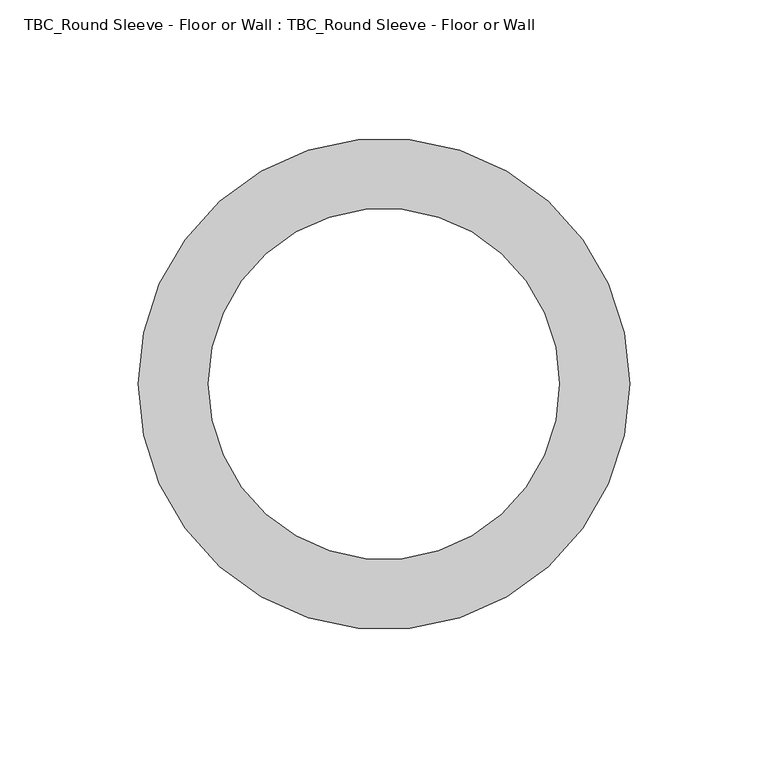
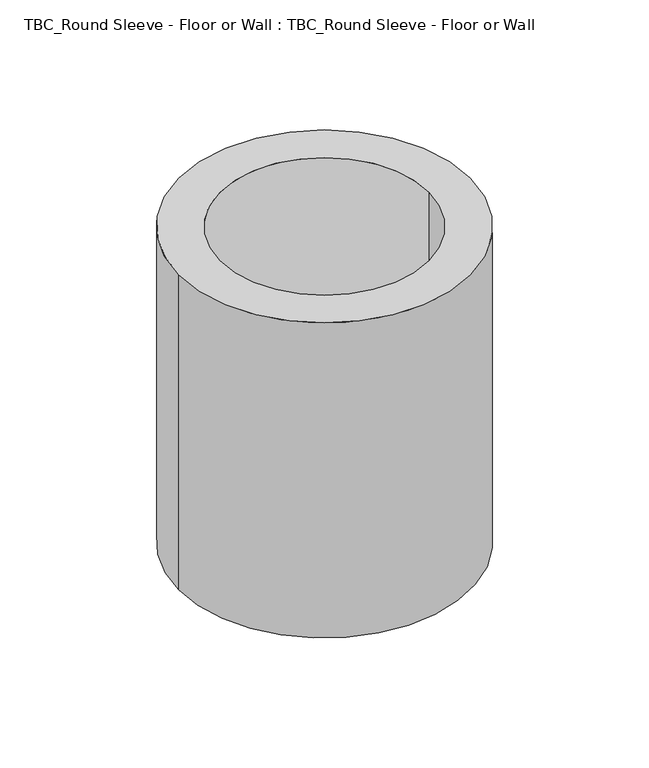
"""IFC4 building model written with IfcOpenShell, lengths in millimetres: proxy geometry, TBC_Round Sleeve - Floor or Wall : TBC_Round Sleeve - Floor or Wall."""

import ifcopenshell
import ifcopenshell.guid

model = None  # the IFC model being written
_history = None  # IfcOwnerHistory: only IFC2X3 demands one
_inside = {}  # id of a spatial element -> (the spatial element, [elements in it])
_under = {}  # id of a project, library or spatial element -> (it, [spatial elements below it])
_declared = {}  # id of a project -> (the project, [libraries it declares])
_typed = {}  # id of a type object -> (the type object, [elements of that type])
_made_of = {}  # id of a material, layer set ... -> (it, [elements and type objects made of it])


def new_model(schema):
    """Start an empty IFC model of exactly this schema.

    Asked for "IFC4X3", IfcOpenShell would pick the latest addendum, in which some entities
    have other attributes; the version numbers below select the first issue.
    IFC2X3 requires an IfcOwnerHistory on every rooted entity: one is made here for all.
    """
    global model, _history
    if schema == "IFC4X3":
        model = ifcopenshell.file(schema_version=(4, 3, 0, 0))
    else:
        model = ifcopenshell.file(schema=schema)
    _inside.clear()
    _under.clear()
    _declared.clear()
    _typed.clear()
    _made_of.clear()
    _history = None
    if model.schema == "IFC2X3":
        org = make("IfcOrganization", Name="unknown")
        user = make(
            "IfcPersonAndOrganization",
            ThePerson=make("IfcPerson", FamilyName="unknown"),
            TheOrganization=org,
        )
        app = make(
            "IfcApplication",
            ApplicationDeveloper=org,
            Version="unknown",
            ApplicationFullName="unknown",
            ApplicationIdentifier="unknown",
        )
        _history = make(
            "IfcOwnerHistory",
            OwningUser=user,
            OwningApplication=app,
            ChangeAction="ADDED",
            CreationDate=0,
        )
    return model


def make(cls, **values):
    """One entity of the class cls with the attributes given. An attribute that is None is left unset."""
    return model.create_entity(
        cls, **{name: value for name, value in values.items() if value is not None}
    )


def rooted(cls, **values):
    """An entity with a GlobalId (a new one), such as an element, a storey or a relation."""
    return make(cls, GlobalId=ifcopenshell.guid.new(), OwnerHistory=_history, **values)


def si_unit(unit_type, name, prefix=None):
    """IfcSIUnit, for example si_unit("LENGTHUNIT", "METRE", prefix="MILLI")."""
    return make("IfcSIUnit", UnitType=unit_type, Prefix=prefix, Name=name)


def assignment(units):
    """IfcUnitAssignment: the units of a project."""
    return None if units is None else make("IfcUnitAssignment", Units=units)


def point(xyz):
    """IfcCartesianPoint."""
    return None if xyz is None else make("IfcCartesianPoint", Coordinates=xyz)


def direction(xyz):
    """IfcDirection."""
    return None if xyz is None else make("IfcDirection", DirectionRatios=xyz)


def frame(location, z_axis=None, x_axis=None):
    """IfcAxis2Placement3D, a coordinate frame: its origin and axes. An axis left out is left unset."""
    return make(
        "IfcAxis2Placement3D",
        Location=point(location),
        Axis=direction(z_axis),
        RefDirection=direction(x_axis),
    )


def frame_2d(location, x_axis=None):
    """IfcAxis2Placement2D, a coordinate frame in the plane: its origin and x axis."""
    return make(
        "IfcAxis2Placement2D", Location=point(location), RefDirection=direction(x_axis)
    )


def origin():
    """The frame at (0, 0, 0) with its axes left unset."""
    return frame((0.0, 0.0, 0.0))


def origin_2d():
    """The frame at (0, 0) in the plane with its x axis left unset."""
    return frame_2d((0.0, 0.0))


def place(relative_to, where):
    """IfcLocalPlacement: puts the frame where relative to a parent placement (None: the world)."""
    return make(
        "IfcLocalPlacement", PlacementRelTo=relative_to, RelativePlacement=where
    )


def context(
    kind, dimensions, precision=None, world=None, true_north=None, identifier=None
):
    """IfcGeometricRepresentationContext, for example the 3D "Model" context."""
    return make(
        "IfcGeometricRepresentationContext",
        ContextIdentifier=identifier,
        ContextType=kind,
        CoordinateSpaceDimension=dimensions,
        Precision=precision,
        WorldCoordinateSystem=world,
        TrueNorth=true_north,
    )


def project(units=None, contexts=None):
    """IfcProject with its units and contexts."""
    return rooted(
        "IfcProject",
        Name="project",
        RepresentationContexts=contexts,
        UnitsInContext=assignment(units),
    )


def spatial(cls, under=None, at=None, **own):
    """A site, building, storey or space (cls), placed at a placement, below another one or the project."""
    s = rooted(cls, ObjectPlacement=at, **own)
    if under is not None:
        _under.setdefault(under.id(), (under, []))[1].append(s)
    return s


def circle_curve(where, radius):
    """IfcCircle in the frame where."""
    return make("IfcCircle", Position=where, Radius=radius)


def trimmed(basis, trim1, trim2, sense, master):
    """IfcTrimmedCurve: the piece of a basis curve between two trims."""
    return make(
        "IfcTrimmedCurve",
        BasisCurve=basis,
        Trim1=trim1,
        Trim2=trim2,
        SenseAgreement=sense,
        MasterRepresentation=master,
    )


def segment(curve, same_sense, transition):
    """IfcCompositeCurveSegment."""
    return make(
        "IfcCompositeCurveSegment",
        Transition=transition,
        SameSense=same_sense,
        ParentCurve=curve,
    )


def composite_curve(segments, self_intersect=None):
    """IfcCompositeCurve: segments joined end to end."""
    return make("IfcCompositeCurve", Segments=segments, SelfIntersect=self_intersect)


def outline(outer, holes=None, kind="AREA"):
    """IfcArbitraryClosedProfileDef: a profile drawn as a closed curve; with holes, ...WithVoids."""
    if holes is None:
        return make("IfcArbitraryClosedProfileDef", ProfileType=kind, OuterCurve=outer)
    return make(
        "IfcArbitraryProfileDefWithVoids",
        ProfileType=kind,
        OuterCurve=outer,
        InnerCurves=holes,
    )


def extrude(swept, where, along, depth):
    """IfcExtrudedAreaSolid: the profile swept, set in the frame where, extruded along a direction by depth."""
    return make(
        "IfcExtrudedAreaSolid",
        SweptArea=swept,
        Position=where,
        ExtrudedDirection=direction(along),
        Depth=depth,
    )


def shape(context_of_items, identifier, shape_type, items):
    """IfcShapeRepresentation: the items that make up one representation, for example the "Body"."""
    return make(
        "IfcShapeRepresentation",
        ContextOfItems=context_of_items,
        RepresentationIdentifier=identifier,
        RepresentationType=shape_type,
        Items=items,
    )


def source(mapping_origin, context_of_items, identifier, shape_type, items):
    """IfcRepresentationMap: a shape defined once, which mapped items show again and again."""
    return make(
        "IfcRepresentationMap",
        MappingOrigin=mapping_origin,
        MappedRepresentation=shape(context_of_items, identifier, shape_type, items),
    )


def transform(
    local_origin,
    x_axis=None,
    y_axis=None,
    z_axis=None,
    scale=None,
    scale2=None,
    scale3=None,
    uniform=True,
):
    """IfcCartesianTransformationOperator3D, or its non-uniform kind. x_axis, y_axis, z_axis: its Axis1, 2, 3."""
    if uniform:
        return make(
            "IfcCartesianTransformationOperator3D",
            Axis1=direction(x_axis),
            Axis2=direction(y_axis),
            LocalOrigin=point(local_origin),
            Scale=scale,
            Axis3=direction(z_axis),
        )
    return make(
        "IfcCartesianTransformationOperator3DnonUniform",
        Axis1=direction(x_axis),
        Axis2=direction(y_axis),
        LocalOrigin=point(local_origin),
        Scale=scale,
        Axis3=direction(z_axis),
        Scale2=scale2,
        Scale3=scale3,
    )


def mapped(mapping_source, mapping_target):
    """IfcMappedItem: shows the shape of a source again, moved by a transform."""
    return make(
        "IfcMappedItem", MappingSource=mapping_source, MappingTarget=mapping_target
    )


def made_of(thing, what):
    """Note that an element or type object is made of a material, layer set ...; save() writes the relation."""
    if what is not None:
        _made_of.setdefault(what.id(), (what, []))[1].append(thing)
    return thing


def element(
    cls,
    number,
    at=None,
    inside=None,
    cuts=None,
    type_object=None,
    material=None,
    context=None,
    identifier="Body",
    shape_type=None,
    held_by="IfcProductDefinitionShape",
    body=None,
    shapes=None,
    **own,
):
    """One element of the class cls, such as IfcWall. Its Tag is "e" and its number.

    at: its placement. inside: the storey or other place that contains it. cuts: it is an
    opening in that element (IfcRelVoidsElement). A single representation is given by context,
    identifier, shape_type and body (its items); several are given by shapes. held_by: the class
    of the entity that holds the representations. save() writes the other relations.
    """
    e = rooted(cls, Tag="e%d" % number, ObjectPlacement=at, **own)
    if body is not None:
        shapes = [shape(context, identifier, shape_type, body)]
    if shapes is not None:
        e.Representation = make(held_by, Representations=shapes)
    if inside is not None:
        _inside.setdefault(inside.id(), (inside, []))[1].append(e)
    if cuts is not None:
        rooted(
            "IfcRelVoidsElement", RelatingBuildingElement=cuts, RelatedOpeningElement=e
        )
    if type_object is not None:
        _typed.setdefault(type_object.id(), (type_object, []))[1].append(e)
    return made_of(e, material)


def aggregate(whole, parts):
    """IfcRelAggregates: a whole, such as a stair, and the parts it consists of."""
    return rooted("IfcRelAggregates", RelatingObject=whole, RelatedObjects=parts)


def save(model, path):
    """Write the relations noted so far, then the file.

    IfcRelAggregates (storeys below a building ...), IfcRelContainedInSpatialStructure (elements
    in a storey), IfcRelDefinesByType, IfcRelAssociatesMaterial and IfcRelDeclares: one each for
    every whole, place, type object, material and project.
    """
    for whole, parts in _under.values():
        aggregate(whole, parts)
    for where, things in _inside.values():
        rooted(
            "IfcRelContainedInSpatialStructure",
            RelatedElements=things,
            RelatingStructure=where,
        )
    for kind, things in _typed.values():
        rooted("IfcRelDefinesByType", RelatedObjects=things, RelatingType=kind)
    for what, things in _made_of.values():
        rooted("IfcRelAssociatesMaterial", RelatedObjects=things, RelatingMaterial=what)
    for by, libraries in _declared.values():
        rooted("IfcRelDeclares", RelatingContext=by, RelatedDefinitions=libraries)
    model.write(path)


def tbc_round_sleeve_floor_or_wall_tbc_round_sleeve_floor_or_aba89356(model_context):
    return source(origin(), model_context, "Body", "SweptSolid", [
        extrude(outline(composite_curve([segment(trimmed(circle_curve(origin_2d(), 88.9), [point((-88.9, 0.0))], [point((88.9, 0.0))], False, "CARTESIAN"), True, "CONTINUOUS"), segment(trimmed(circle_curve(origin_2d(), 88.9), [point((88.9, 0.0))], [point((-88.9, 0.0))], False, "CARTESIAN"), True, "CONTINUOUS")], self_intersect=False), holes=[composite_curve([segment(trimmed(circle_curve(origin_2d(), 63.5), [point((-63.5, 0.0))], [point((63.5, 0.0))], True, "CARTESIAN"), True, "CONTINUOUS"), segment(trimmed(circle_curve(origin_2d(), 63.5), [point((63.5, 0.0))], [point((-63.5, 0.0))], True, "CARTESIAN"), True, "CONTINUOUS")], self_intersect=False)]), frame((0.0, 0.0, -203.2), z_axis=(0.0, 0.0, 1.0), x_axis=(1.0, 0.0, 0.0)), (0.0, 0.0, 1.0), 203.2),
    ])


if __name__ == "__main__":
    model = new_model("IFC4")
    model_context = context("Model", 3, world=origin())
    ifc_project = project(units=[si_unit("LENGTHUNIT", "METRE", prefix="MILLI")], contexts=[model_context])
    site = spatial("IfcSite", under=ifc_project)
    building = spatial("IfcBuilding", under=site)
    placement = place(None, origin())
    tbc_round_sleeve_floor_or_wall_tbc_round_sleeve_floor_or_shape = tbc_round_sleeve_floor_or_wall_tbc_round_sleeve_floor_or_aba89356(model_context)
    element("IfcBuildingElementProxy", 1, Name="TBC_Round Sleeve - Floor or Wall : TBC_Round Sleeve - Floor or Wall", ObjectType="TBC_Round Sleeve - Floor or Wall : TBC_Round Sleeve - Floor or Wall", at=placement, inside=building, context=model_context, shape_type="MappedRepresentation", body=[
        mapped(tbc_round_sleeve_floor_or_wall_tbc_round_sleeve_floor_or_shape, transform((0.0, 0.0, 0.0), x_axis=(1.0, 0.0, 0.0), y_axis=(0.0, 1.0, 0.0), z_axis=(0.0, 0.0, 1.0))),
    ])
    save(model, "model.ifc")

# Revit data of these elements
# Type "TBC_Round Sleeve - Floor or Wall : TBC_Round Sleeve - Floor or Wall"
#   Tag Dimension [instance default] = ""
#   MEP Type [instance default] = ""
#   MEP Element [instance default] = ""
#   MEP Category [instance default] = ""
#   Host Element Type [instance default] = ""
#   Host Element Id [instance default] = ""
#   Host Element Category [instance default] = ""
#   Control Line Y [instance default] = ""
#   Control Line X [instance default] = ""
#   Sleeve Radius [instance default] = 1' - 0"
#   Sleeve Edge [instance default] = 1' - 2"
#   Sleeve Depth [instance default] = 3' - 0"
#   Distance Y [instance default] = 0' - 0"
#   Distance X [instance default] = 0' - 0"
#   Default Elevation = 0
# Element 1 (IfcBuildingElementProxy, "TBC_Round Sleeve - Floor or Wall : TBC_Round Sleeve - Floor or Wall")
#   MEP Type = "PLG-ST"
#   MEP Element = "828943"
#   MEP Category = "Pipe"
#   Host Element Type = "8\" Plank"
#   Host Element Id = "529506"
#   Host Element Category = "Floors"
#   Sleeve Radius = 0' - 5"
#   Sleeve Edge = 0' - 7"
#   Sleeve Depth = 0' - 8"
